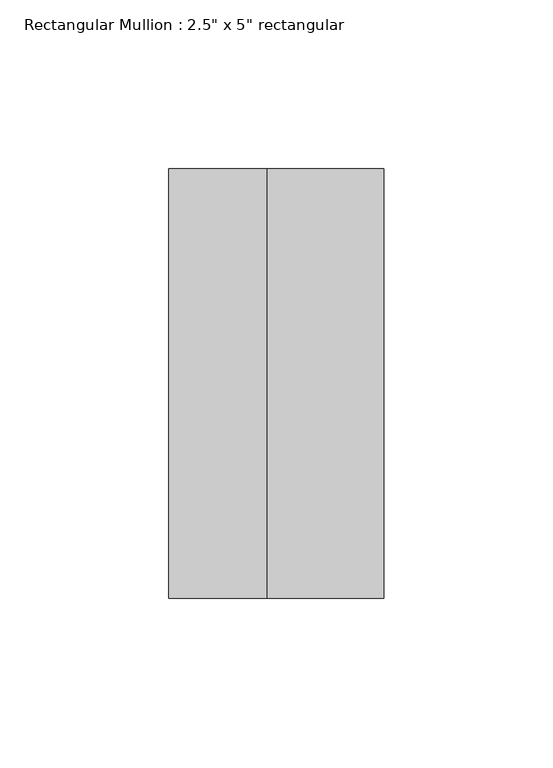
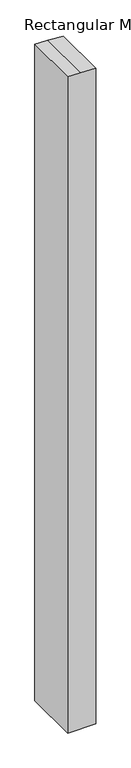
"""IFC4 building model written with IfcOpenShell, lengths in millimetres: member geometry."""

import ifcopenshell
import ifcopenshell.guid

model = None  # the IFC model being written
_history = None  # IfcOwnerHistory: only IFC2X3 demands one
_inside = {}  # id of a spatial element -> (the spatial element, [elements in it])
_under = {}  # id of a project, library or spatial element -> (it, [spatial elements below it])
_declared = {}  # id of a project -> (the project, [libraries it declares])
_typed = {}  # id of a type object -> (the type object, [elements of that type])
_made_of = {}  # id of a material, layer set ... -> (it, [elements and type objects made of it])


def new_model(schema):
    """Start an empty IFC model of exactly this schema.

    Asked for "IFC4X3", IfcOpenShell would pick the latest addendum, in which some entities
    have other attributes; the version numbers below select the first issue.
    IFC2X3 requires an IfcOwnerHistory on every rooted entity: one is made here for all.
    """
    global model, _history
    if schema == "IFC4X3":
        model = ifcopenshell.file(schema_version=(4, 3, 0, 0))
    else:
        model = ifcopenshell.file(schema=schema)
    _inside.clear()
    _under.clear()
    _declared.clear()
    _typed.clear()
    _made_of.clear()
    _history = None
    if model.schema == "IFC2X3":
        org = make("IfcOrganization", Name="unknown")
        user = make(
            "IfcPersonAndOrganization",
            ThePerson=make("IfcPerson", FamilyName="unknown"),
            TheOrganization=org,
        )
        app = make(
            "IfcApplication",
            ApplicationDeveloper=org,
            Version="unknown",
            ApplicationFullName="unknown",
            ApplicationIdentifier="unknown",
        )
        _history = make(
            "IfcOwnerHistory",
            OwningUser=user,
            OwningApplication=app,
            ChangeAction="ADDED",
            CreationDate=0,
        )
    return model


def make(cls, **values):
    """One entity of the class cls with the attributes given. An attribute that is None is left unset."""
    return model.create_entity(
        cls, **{name: value for name, value in values.items() if value is not None}
    )


def rooted(cls, **values):
    """An entity with a GlobalId (a new one), such as an element, a storey or a relation."""
    return make(cls, GlobalId=ifcopenshell.guid.new(), OwnerHistory=_history, **values)


def si_unit(unit_type, name, prefix=None):
    """IfcSIUnit, for example si_unit("LENGTHUNIT", "METRE", prefix="MILLI")."""
    return make("IfcSIUnit", UnitType=unit_type, Prefix=prefix, Name=name)


def assignment(units):
    """IfcUnitAssignment: the units of a project."""
    return None if units is None else make("IfcUnitAssignment", Units=units)


def point(xyz):
    """IfcCartesianPoint."""
    return None if xyz is None else make("IfcCartesianPoint", Coordinates=xyz)


def direction(xyz):
    """IfcDirection."""
    return None if xyz is None else make("IfcDirection", DirectionRatios=xyz)


def frame(location, z_axis=None, x_axis=None):
    """IfcAxis2Placement3D, a coordinate frame: its origin and axes. An axis left out is left unset."""
    return make(
        "IfcAxis2Placement3D",
        Location=point(location),
        Axis=direction(z_axis),
        RefDirection=direction(x_axis),
    )


def origin():
    """The frame at (0, 0, 0) with its axes left unset."""
    return frame((0.0, 0.0, 0.0))


def place(relative_to, where):
    """IfcLocalPlacement: puts the frame where relative to a parent placement (None: the world)."""
    return make(
        "IfcLocalPlacement", PlacementRelTo=relative_to, RelativePlacement=where
    )


def context(
    kind, dimensions, precision=None, world=None, true_north=None, identifier=None
):
    """IfcGeometricRepresentationContext, for example the 3D "Model" context."""
    return make(
        "IfcGeometricRepresentationContext",
        ContextIdentifier=identifier,
        ContextType=kind,
        CoordinateSpaceDimension=dimensions,
        Precision=precision,
        WorldCoordinateSystem=world,
        TrueNorth=true_north,
    )


def project(units=None, contexts=None):
    """IfcProject with its units and contexts."""
    return rooted(
        "IfcProject",
        Name="project",
        RepresentationContexts=contexts,
        UnitsInContext=assignment(units),
    )


def spatial(cls, under=None, at=None, **own):
    """A site, building, storey or space (cls), placed at a placement, below another one or the project."""
    s = rooted(cls, ObjectPlacement=at, **own)
    if under is not None:
        _under.setdefault(under.id(), (under, []))[1].append(s)
    return s


def polyline(points):
    """IfcPolyline through the points."""
    return make("IfcPolyline", Points=[point(p) for p in points])


def outline(outer, holes=None, kind="AREA"):
    """IfcArbitraryClosedProfileDef: a profile drawn as a closed curve; with holes, ...WithVoids."""
    if holes is None:
        return make("IfcArbitraryClosedProfileDef", ProfileType=kind, OuterCurve=outer)
    return make(
        "IfcArbitraryProfileDefWithVoids",
        ProfileType=kind,
        OuterCurve=outer,
        InnerCurves=holes,
    )


def extrude(swept, where, along, depth):
    """IfcExtrudedAreaSolid: the profile swept, set in the frame where, extruded along a direction by depth."""
    return make(
        "IfcExtrudedAreaSolid",
        SweptArea=swept,
        Position=where,
        ExtrudedDirection=direction(along),
        Depth=depth,
    )


def shape(context_of_items, identifier, shape_type, items):
    """IfcShapeRepresentation: the items that make up one representation, for example the "Body"."""
    return make(
        "IfcShapeRepresentation",
        ContextOfItems=context_of_items,
        RepresentationIdentifier=identifier,
        RepresentationType=shape_type,
        Items=items,
    )


def source(mapping_origin, context_of_items, identifier, shape_type, items):
    """IfcRepresentationMap: a shape defined once, which mapped items show again and again."""
    return make(
        "IfcRepresentationMap",
        MappingOrigin=mapping_origin,
        MappedRepresentation=shape(context_of_items, identifier, shape_type, items),
    )


def transform(
    local_origin,
    x_axis=None,
    y_axis=None,
    z_axis=None,
    scale=None,
    scale2=None,
    scale3=None,
    uniform=True,
):
    """IfcCartesianTransformationOperator3D, or its non-uniform kind. x_axis, y_axis, z_axis: its Axis1, 2, 3."""
    if uniform:
        return make(
            "IfcCartesianTransformationOperator3D",
            Axis1=direction(x_axis),
            Axis2=direction(y_axis),
            LocalOrigin=point(local_origin),
            Scale=scale,
            Axis3=direction(z_axis),
        )
    return make(
        "IfcCartesianTransformationOperator3DnonUniform",
        Axis1=direction(x_axis),
        Axis2=direction(y_axis),
        LocalOrigin=point(local_origin),
        Scale=scale,
        Axis3=direction(z_axis),
        Scale2=scale2,
        Scale3=scale3,
    )


def mapped(mapping_source, mapping_target):
    """IfcMappedItem: shows the shape of a source again, moved by a transform."""
    return make(
        "IfcMappedItem", MappingSource=mapping_source, MappingTarget=mapping_target
    )


def made_of(thing, what):
    """Note that an element or type object is made of a material, layer set ...; save() writes the relation."""
    if what is not None:
        _made_of.setdefault(what.id(), (what, []))[1].append(thing)
    return thing


def element(
    cls,
    number,
    at=None,
    inside=None,
    cuts=None,
    type_object=None,
    material=None,
    context=None,
    identifier="Body",
    shape_type=None,
    held_by="IfcProductDefinitionShape",
    body=None,
    shapes=None,
    **own,
):
    """One element of the class cls, such as IfcWall. Its Tag is "e" and its number.

    at: its placement. inside: the storey or other place that contains it. cuts: it is an
    opening in that element (IfcRelVoidsElement). A single representation is given by context,
    identifier, shape_type and body (its items); several are given by shapes. held_by: the class
    of the entity that holds the representations. save() writes the other relations.
    """
    e = rooted(cls, Tag="e%d" % number, ObjectPlacement=at, **own)
    if body is not None:
        shapes = [shape(context, identifier, shape_type, body)]
    if shapes is not None:
        e.Representation = make(held_by, Representations=shapes)
    if inside is not None:
        _inside.setdefault(inside.id(), (inside, []))[1].append(e)
    if cuts is not None:
        rooted(
            "IfcRelVoidsElement", RelatingBuildingElement=cuts, RelatedOpeningElement=e
        )
    if type_object is not None:
        _typed.setdefault(type_object.id(), (type_object, []))[1].append(e)
    return made_of(e, material)


def aggregate(whole, parts):
    """IfcRelAggregates: a whole, such as a stair, and the parts it consists of."""
    return rooted("IfcRelAggregates", RelatingObject=whole, RelatedObjects=parts)


def save(model, path):
    """Write the relations noted so far, then the file.

    IfcRelAggregates (storeys below a building ...), IfcRelContainedInSpatialStructure (elements
    in a storey), IfcRelDefinesByType, IfcRelAssociatesMaterial and IfcRelDeclares: one each for
    every whole, place, type object, material and project.
    """
    for whole, parts in _under.values():
        aggregate(whole, parts)
    for where, things in _inside.values():
        rooted(
            "IfcRelContainedInSpatialStructure",
            RelatedElements=things,
            RelatingStructure=where,
        )
    for kind, things in _typed.values():
        rooted("IfcRelDefinesByType", RelatedObjects=things, RelatingType=kind)
    for what, things in _made_of.values():
        rooted("IfcRelAssociatesMaterial", RelatedObjects=things, RelatingMaterial=what)
    for by, libraries in _declared.values():
        rooted("IfcRelDeclares", RelatingContext=by, RelatedDefinitions=libraries)
    model.write(path)


def member_a00ec9cd(model_context):
    return source(origin(), model_context, "Body", "SweptSolid", [
        extrude(outline(polyline([(-64.8775557, 31.75), (-63.4449853, -2.6426951), (-62.232569, -31.75), (-1619.8278232, -31.75), (-1619.8278232, 31.75), (-64.8775557, 31.75)])), frame((0.0, -63.5, 0.0), z_axis=(0.0, 1.0, 0.0), x_axis=(0.0, 0.0, 1.0)), (0.0, 0.0, 1.0), 127.0),
    ])


if __name__ == "__main__":
    model = new_model("IFC4")
    model_context = context("Model", 3, world=origin())
    ifc_project = project(units=[si_unit("LENGTHUNIT", "METRE", prefix="MILLI")], contexts=[model_context])
    site = spatial("IfcSite", under=ifc_project)
    building = spatial("IfcBuilding", under=site)
    placement = place(None, origin())
    member_shape = member_a00ec9cd(model_context)
    element("IfcMember", 1, ObjectType="Rectangular Mullion : 2.5\" x 5\" rectangular", at=placement, inside=building, context=model_context, shape_type="MappedRepresentation", body=[
        mapped(member_shape, transform((0.0, 0.0, 0.0), x_axis=(1.0, 0.0, 0.0), y_axis=(0.0, 1.0, 0.0), z_axis=(0.0, 0.0, 1.0))),
    ])
    save(model, "model.ifc")

# Revit data of these elements
# Type "Rectangular Mullion : 2.5\" x 5\" rectangular"
#   built-in parameter 1007304 = 0.416667 (stored number, unit not read)
#   built-in parameter 1007301 = 0.104167 (stored number, unit not read)
#   built-in parameter 1007300 = 0.104167 (stored number, unit not read)
# Element 1 (IfcMember, "Rectangular Mullion : 2.5\" x 5\" rectangular")
#   Materials on its faces: "Aluminum"
# Materials
#   "Aluminum": class "Metal", colour RGB 247 247 247, transparency 0, Description = "Aluminum 6061", Cost = 0
